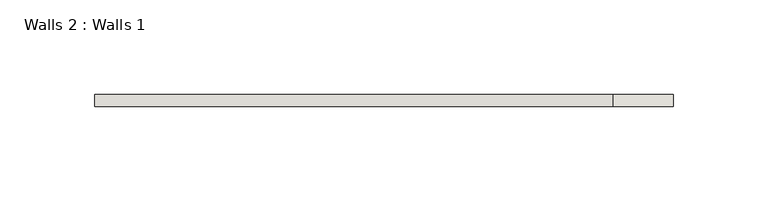
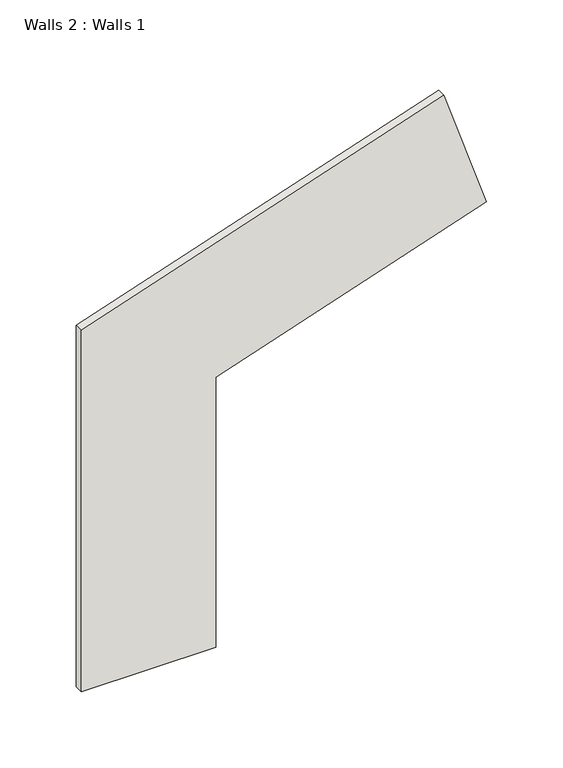
"""IFC4 building model written with IfcOpenShell, lengths in millimetres: wall geometry, Walls 2 : Walls 1."""

from ifc_helpers import new_model, si_unit, frame, origin, place, context, project, spatial, polyline, outline, extrude, source, transform, mapped, element, save


def walls_2_walls_1_5fe68988(model_context):
    return source(origin(), model_context, "Body", "SweptSolid", [
        extrude(outline(polyline([(5071.1413299, 19768.3370052), (4782.1134335, 19768.3370052), (4782.1134335, 19869.9370052), (4998.0134335, 19869.9370052), (5066.5557127, 20074.6679651), (5162.8996939, 20042.4127749), (5071.1413299, 19768.3370052)])), frame((0.0, -1122.6884634, 0.0), z_axis=(0.0, 1.0, 0.0), x_axis=(0.0, 0.0, 1.0)), (0.0, 0.0, 1.0), 6.35),
    ])


if __name__ == "__main__":
    model = new_model("IFC4")
    model_context = context("Model", 3, world=origin())
    ifc_project = project(units=[si_unit("LENGTHUNIT", "METRE", prefix="MILLI")], contexts=[model_context])
    site = spatial("IfcSite", under=ifc_project)
    building = spatial("IfcBuilding", under=site)
    placement = place(None, origin())
    walls_2_walls_1_shape = walls_2_walls_1_5fe68988(model_context)
    element("IfcWall", 1, ObjectType="Walls 2 : Walls 1", at=placement, inside=building, context=model_context, shape_type="MappedRepresentation", body=[
        mapped(walls_2_walls_1_shape, transform((0.0, 0.0, 0.0), x_axis=(1.0, 0.0, 0.0), y_axis=(0.0, 1.0, 0.0), z_axis=(0.0, 0.0, 1.0))),
    ])
    save(model, "model.ifc")

# Revit data of these elements
# Element 1 (IfcWall, "Walls 2 : Walls 1")
#   Materials on its faces: "1/4\" STEEL GUSSET PLATE - (RAW STEEL)"
# Materials
#   "1/4\" STEEL GUSSET PLATE - (RAW STEEL)": class "Metal", colour RGB 189 187 185, transparency 0, Description = "Structural steel 50ksi", Cost = 0
